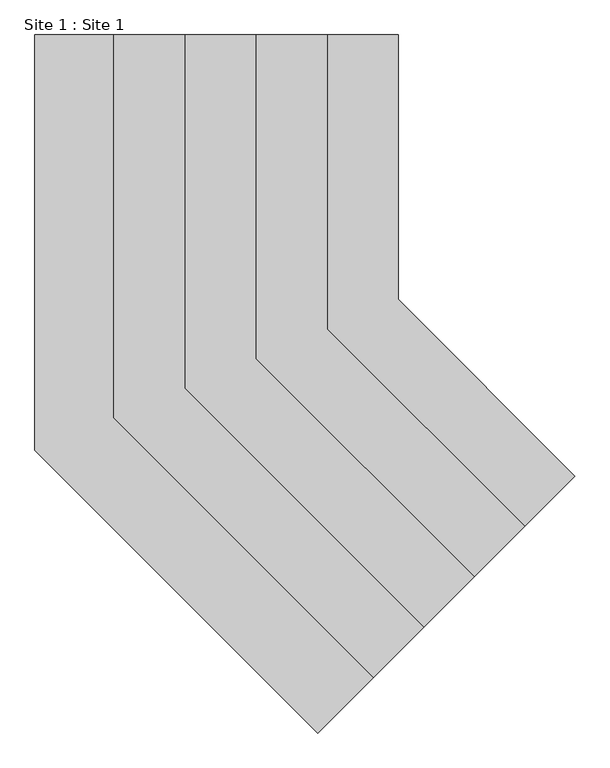
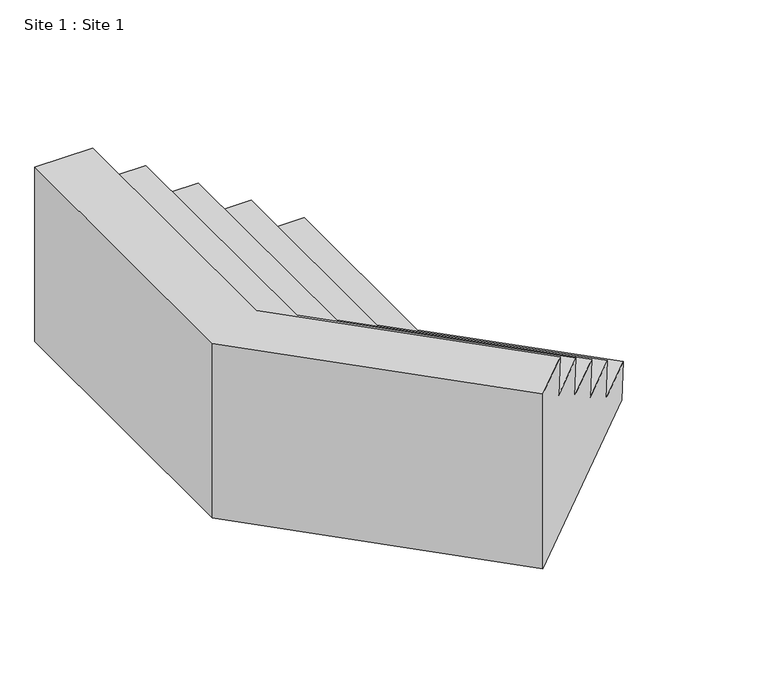
"""IFC4 building model written with IfcOpenShell, lengths in millimetres: geographic element geometry, Site 1 : Site 1."""

from ifc_helpers import new_model, si_unit, origin, place, context, project, spatial, faceted_brep, source, transform, mapped, element, save


def site_1_site_1_ca4687d6(model_context):
    return source(origin(), model_context, "Body", "Brep", [
        faceted_brep([(31305.1418347, 23210.4968756, 264845.4280751), (31107.5762, 23012.9312409, 264845.4280751), (31107.5762, 23012.9312409, 263956.4280751), (32005.6018121, 23910.956853, 263956.4280751), (32023.5623243, 23928.9173652, 264134.2280751), (31825.9966897, 23731.3517306, 264134.2280751), (31843.9572019, 23749.3122428, 264312.0280751), (31646.3915673, 23551.7466082, 264312.0280751), (31664.3520795, 23569.7071204, 264489.8280751), (31466.7864448, 23372.1414857, 264489.8280751), (31484.7469571, 23390.101998, 264667.6280751), (31287.1813224, 23192.5363633, 264667.6280751), (30378.5088966, 24137.1298137, 264845.4280751), (30378.5088966, 25500.6656612, 264845.4280751), (30099.1088966, 25500.6656612, 264845.4280751), (30099.1088966, 24021.3985443, 264845.4280751), (30099.1088966, 24021.3985443, 263956.4280751), (30099.1088966, 25500.6656612, 263956.4280751), (31369.1088966, 25500.6656612, 263956.4280751), (31369.1088966, 24547.4497686, 263956.4280751), (31394.5088966, 24557.970793, 264134.2280751), (31394.5088966, 25500.6656612, 264134.2280751), (31115.1088966, 25500.6656612, 264134.2280751), (31115.1088966, 24442.2395237, 264134.2280751), (31140.5088966, 24452.7605482, 264312.0280751), (31140.5088966, 25500.6656612, 264312.0280751), (30861.1088966, 25500.6656612, 264312.0280751), (30861.1088966, 24337.0292789, 264312.0280751), (30886.5088966, 24347.5503034, 264489.8280751), (30886.5088966, 25500.6656612, 264489.8280751), (30607.1088966, 25500.6656612, 264489.8280751), (30607.1088966, 24231.819034, 264489.8280751), (30632.5088966, 24242.3400585, 264667.6280751), (30632.5088966, 25500.6656612, 264667.6280751), (30353.1088966, 25500.6656612, 264667.6280751), (30353.1088966, 24126.6087892, 264667.6280751)], [[[0, 1, 2, 3, 4, 5, 6, 7, 8, 9, 10, 11]], [[1, 0, 12, 13, 14, 15]], [[2, 1, 15, 16]], [[3, 2, 16, 17, 18, 19]], [[4, 3, 19, 20]], [[5, 4, 20, 21, 22, 23]], [[6, 5, 23, 24]], [[7, 6, 24, 25, 26, 27]], [[8, 7, 27, 28]], [[9, 8, 28, 29, 30, 31]], [[10, 9, 31, 32]], [[11, 10, 32, 33, 34, 35]], [[0, 11, 35, 12]], [[13, 34, 33, 30, 29, 26, 25, 22, 21, 18, 17, 14]], [[16, 15, 14, 17]], [[20, 19, 18, 21]], [[24, 23, 22, 25]], [[28, 27, 26, 29]], [[32, 31, 30, 33]], [[12, 35, 34, 13]]]),
    ])


if __name__ == "__main__":
    model = new_model("IFC4")
    model_context = context("Model", 3, world=origin())
    ifc_project = project(units=[si_unit("LENGTHUNIT", "METRE", prefix="MILLI")], contexts=[model_context])
    site = spatial("IfcSite", under=ifc_project)
    building = spatial("IfcBuilding", under=site)
    placement = place(None, origin())
    site_1_site_1_shape = site_1_site_1_ca4687d6(model_context)
    element("IfcGeographicElement", 1, ObjectType="Site 1 : Site 1", at=placement, inside=building, context=model_context, shape_type="MappedRepresentation", body=[
        mapped(site_1_site_1_shape, transform((0.0, 0.0, 0.0), x_axis=(1.0, 0.0, 0.0), y_axis=(0.0, 1.0, 0.0), z_axis=(0.0, 0.0, 1.0))),
    ])
    save(model, "model.ifc")

# Revit data of these elements
# Element 1 (IfcGeographicElement, "Site 1 : Site 1")
#   Materials on its faces: "Sidewalk"
# Materials
#   "Sidewalk": class "Concrete", colour RGB 255 255 255, transparency 0, Description = "Cast-in-place concrete", Cost = 0
